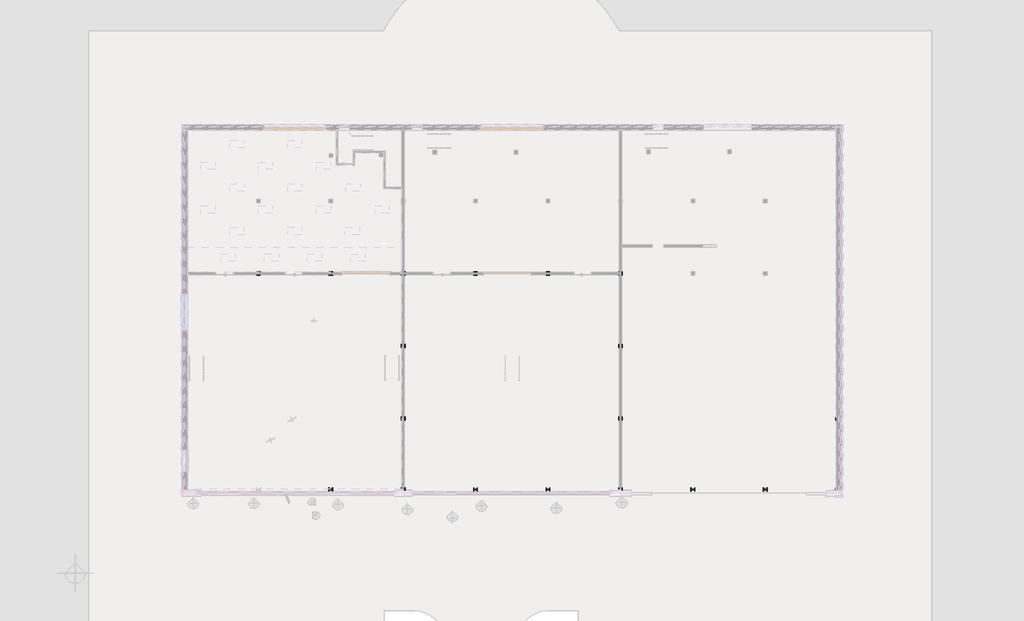
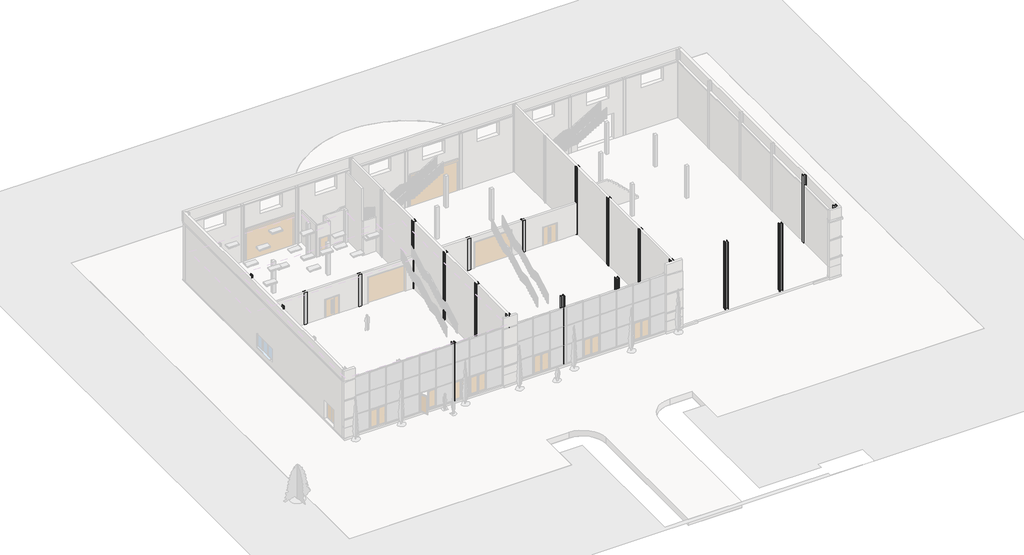
# One storey, part 5 of 13: 21 columns, 21 slabs, 8 footings.
"""IFC4 building model written with IfcOpenShell, lengths in millimetres."""

import ifcopenshell
import ifcopenshell.guid

model = None  # the IFC model being written
_history = None  # IfcOwnerHistory: only IFC2X3 demands one
_inside = {}  # id of a spatial element -> (the spatial element, [elements in it])
_under = {}  # id of a project, library or spatial element -> (it, [spatial elements below it])
_declared = {}  # id of a project -> (the project, [libraries it declares])
_typed = {}  # id of a type object -> (the type object, [elements of that type])
_made_of = {}  # id of a material, layer set ... -> (it, [elements and type objects made of it])


def new_model(schema):
    """Start an empty IFC model of exactly this schema.

    Asked for "IFC4X3", IfcOpenShell would pick the latest addendum, in which some entities
    have other attributes; the version numbers below select the first issue.
    IFC2X3 requires an IfcOwnerHistory on every rooted entity: one is made here for all.
    """
    global model, _history
    if schema == "IFC4X3":
        model = ifcopenshell.file(schema_version=(4, 3, 0, 0))
    else:
        model = ifcopenshell.file(schema=schema)
    _inside.clear()
    _under.clear()
    _declared.clear()
    _typed.clear()
    _made_of.clear()
    _history = None
    if model.schema == "IFC2X3":
        org = make("IfcOrganization", Name="unknown")
        user = make(
            "IfcPersonAndOrganization",
            ThePerson=make("IfcPerson", FamilyName="unknown"),
            TheOrganization=org,
        )
        app = make(
            "IfcApplication",
            ApplicationDeveloper=org,
            Version="unknown",
            ApplicationFullName="unknown",
            ApplicationIdentifier="unknown",
        )
        _history = make(
            "IfcOwnerHistory",
            OwningUser=user,
            OwningApplication=app,
            ChangeAction="ADDED",
            CreationDate=0,
        )
    return model


def make(cls, **values):
    """One entity of the class cls with the attributes given. An attribute that is None is left unset."""
    return model.create_entity(
        cls, **{name: value for name, value in values.items() if value is not None}
    )


def rooted(cls, **values):
    """An entity with a GlobalId (a new one), such as an element, a storey or a relation."""
    return make(cls, GlobalId=ifcopenshell.guid.new(), OwnerHistory=_history, **values)


def si_unit(unit_type, name, prefix=None):
    """IfcSIUnit, for example si_unit("LENGTHUNIT", "METRE", prefix="MILLI")."""
    return make("IfcSIUnit", UnitType=unit_type, Prefix=prefix, Name=name)


def assignment(units):
    """IfcUnitAssignment: the units of a project."""
    return None if units is None else make("IfcUnitAssignment", Units=units)


def point(xyz):
    """IfcCartesianPoint."""
    return None if xyz is None else make("IfcCartesianPoint", Coordinates=xyz)


def direction(xyz):
    """IfcDirection."""
    return None if xyz is None else make("IfcDirection", DirectionRatios=xyz)


def frame(location, z_axis=None, x_axis=None):
    """IfcAxis2Placement3D, a coordinate frame: its origin and axes. An axis left out is left unset."""
    return make(
        "IfcAxis2Placement3D",
        Location=point(location),
        Axis=direction(z_axis),
        RefDirection=direction(x_axis),
    )


def frame_2d(location, x_axis=None):
    """IfcAxis2Placement2D, a coordinate frame in the plane: its origin and x axis."""
    return make(
        "IfcAxis2Placement2D", Location=point(location), RefDirection=direction(x_axis)
    )


def origin():
    """The frame at (0, 0, 0) with its axes left unset."""
    return frame((0.0, 0.0, 0.0))


def place(relative_to, where):
    """IfcLocalPlacement: puts the frame where relative to a parent placement (None: the world)."""
    return make(
        "IfcLocalPlacement", PlacementRelTo=relative_to, RelativePlacement=where
    )


def context(
    kind, dimensions, precision=None, world=None, true_north=None, identifier=None
):
    """IfcGeometricRepresentationContext, for example the 3D "Model" context."""
    return make(
        "IfcGeometricRepresentationContext",
        ContextIdentifier=identifier,
        ContextType=kind,
        CoordinateSpaceDimension=dimensions,
        Precision=precision,
        WorldCoordinateSystem=world,
        TrueNorth=true_north,
    )


def project(units=None, contexts=None):
    """IfcProject with its units and contexts."""
    return rooted(
        "IfcProject",
        Name="project",
        RepresentationContexts=contexts,
        UnitsInContext=assignment(units),
    )


def spatial(cls, under=None, at=None, **own):
    """A site, building, storey or space (cls), placed at a placement, below another one or the project."""
    s = rooted(cls, ObjectPlacement=at, **own)
    if under is not None:
        _under.setdefault(under.id(), (under, []))[1].append(s)
    return s


def polyline(points):
    """IfcPolyline through the points."""
    return make("IfcPolyline", Points=[point(p) for p in points])


def circle_curve(where, radius):
    """IfcCircle in the frame where."""
    return make("IfcCircle", Position=where, Radius=radius)


def trimmed(basis, trim1, trim2, sense, master):
    """IfcTrimmedCurve: the piece of a basis curve between two trims."""
    return make(
        "IfcTrimmedCurve",
        BasisCurve=basis,
        Trim1=trim1,
        Trim2=trim2,
        SenseAgreement=sense,
        MasterRepresentation=master,
    )


def segment(curve, same_sense, transition):
    """IfcCompositeCurveSegment."""
    return make(
        "IfcCompositeCurveSegment",
        Transition=transition,
        SameSense=same_sense,
        ParentCurve=curve,
    )


def composite_curve(segments, self_intersect=None):
    """IfcCompositeCurve: segments joined end to end."""
    return make("IfcCompositeCurve", Segments=segments, SelfIntersect=self_intersect)


def outline(outer, holes=None, kind="AREA"):
    """IfcArbitraryClosedProfileDef: a profile drawn as a closed curve; with holes, ...WithVoids."""
    if holes is None:
        return make("IfcArbitraryClosedProfileDef", ProfileType=kind, OuterCurve=outer)
    return make(
        "IfcArbitraryProfileDefWithVoids",
        ProfileType=kind,
        OuterCurve=outer,
        InnerCurves=holes,
    )


def extrude(swept, where, along, depth):
    """IfcExtrudedAreaSolid: the profile swept, set in the frame where, extruded along a direction by depth."""
    return make(
        "IfcExtrudedAreaSolid",
        SweptArea=swept,
        Position=where,
        ExtrudedDirection=direction(along),
        Depth=depth,
    )


def faces_of(points, faces, orient=None, outer=None):
    """IfcFace entities. A face is a list of loops; a loop is a list of indices into points, from 0.

    orient and outer hold one flag for each loop. By default every Orientation is true, the
    first loop of a face is its IfcFaceOuterBound and the others are IfcFaceBound.
    """
    made = []
    for i, loops in enumerate(faces):
        bounds = []
        for j, loop in enumerate(loops):
            is_outer = j == 0 if outer is None else outer[i][j]
            bounds.append(
                make(
                    "IfcFaceOuterBound" if is_outer else "IfcFaceBound",
                    Bound=make("IfcPolyLoop", Polygon=[points[k] for k in loop]),
                    Orientation=True if orient is None else orient[i][j],
                )
            )
        made.append(make("IfcFace", Bounds=bounds))
    return made


def faceted_brep(points, faces, orient=None, outer=None, voids=None):
    """IfcFacetedBrep: a solid bounded by flat faces; with voids (closed shells), ...WithVoids."""
    shared = [point(p) for p in points]
    hull = make("IfcClosedShell", CfsFaces=faces_of(shared, faces, orient, outer))
    if voids is None:
        return make("IfcFacetedBrep", Outer=hull)
    return make(
        "IfcFacetedBrepWithVoids",
        Outer=hull,
        Voids=[
            make(cls, CfsFaces=faces_of(shared, fs, o, b)) for cls, fs, o, b in voids
        ],
    )


def shape(context_of_items, identifier, shape_type, items):
    """IfcShapeRepresentation: the items that make up one representation, for example the "Body"."""
    return make(
        "IfcShapeRepresentation",
        ContextOfItems=context_of_items,
        RepresentationIdentifier=identifier,
        RepresentationType=shape_type,
        Items=items,
    )


def source(mapping_origin, context_of_items, identifier, shape_type, items):
    """IfcRepresentationMap: a shape defined once, which mapped items show again and again."""
    return make(
        "IfcRepresentationMap",
        MappingOrigin=mapping_origin,
        MappedRepresentation=shape(context_of_items, identifier, shape_type, items),
    )


def transform(
    local_origin,
    x_axis=None,
    y_axis=None,
    z_axis=None,
    scale=None,
    scale2=None,
    scale3=None,
    uniform=True,
):
    """IfcCartesianTransformationOperator3D, or its non-uniform kind. x_axis, y_axis, z_axis: its Axis1, 2, 3."""
    if uniform:
        return make(
            "IfcCartesianTransformationOperator3D",
            Axis1=direction(x_axis),
            Axis2=direction(y_axis),
            LocalOrigin=point(local_origin),
            Scale=scale,
            Axis3=direction(z_axis),
        )
    return make(
        "IfcCartesianTransformationOperator3DnonUniform",
        Axis1=direction(x_axis),
        Axis2=direction(y_axis),
        LocalOrigin=point(local_origin),
        Scale=scale,
        Axis3=direction(z_axis),
        Scale2=scale2,
        Scale3=scale3,
    )


def mapped(mapping_source, mapping_target):
    """IfcMappedItem: shows the shape of a source again, moved by a transform."""
    return make(
        "IfcMappedItem", MappingSource=mapping_source, MappingTarget=mapping_target
    )


def made_of(thing, what):
    """Note that an element or type object is made of a material, layer set ...; save() writes the relation."""
    if what is not None:
        _made_of.setdefault(what.id(), (what, []))[1].append(thing)
    return thing


def element(
    cls,
    number,
    at=None,
    inside=None,
    cuts=None,
    type_object=None,
    material=None,
    context=None,
    identifier="Body",
    shape_type=None,
    held_by="IfcProductDefinitionShape",
    body=None,
    shapes=None,
    **own,
):
    """One element of the class cls, such as IfcWall. Its Tag is "e" and its number.

    at: its placement. inside: the storey or other place that contains it. cuts: it is an
    opening in that element (IfcRelVoidsElement). A single representation is given by context,
    identifier, shape_type and body (its items); several are given by shapes. held_by: the class
    of the entity that holds the representations. save() writes the other relations.
    """
    e = rooted(cls, Tag="e%d" % number, ObjectPlacement=at, **own)
    if body is not None:
        shapes = [shape(context, identifier, shape_type, body)]
    if shapes is not None:
        e.Representation = make(held_by, Representations=shapes)
    if inside is not None:
        _inside.setdefault(inside.id(), (inside, []))[1].append(e)
    if cuts is not None:
        rooted(
            "IfcRelVoidsElement", RelatingBuildingElement=cuts, RelatedOpeningElement=e
        )
    if type_object is not None:
        _typed.setdefault(type_object.id(), (type_object, []))[1].append(e)
    return made_of(e, material)


def aggregate(whole, parts):
    """IfcRelAggregates: a whole, such as a stair, and the parts it consists of."""
    return rooted("IfcRelAggregates", RelatingObject=whole, RelatedObjects=parts)


def save(model, path):
    """Write the relations noted so far, then the file.

    IfcRelAggregates (storeys below a building ...), IfcRelContainedInSpatialStructure (elements
    in a storey), IfcRelDefinesByType, IfcRelAssociatesMaterial and IfcRelDeclares: one each for
    every whole, place, type object, material and project.
    """
    for whole, parts in _under.values():
        aggregate(whole, parts)
    for where, things in _inside.values():
        rooted(
            "IfcRelContainedInSpatialStructure",
            RelatedElements=things,
            RelatingStructure=where,
        )
    for kind, things in _typed.values():
        rooted("IfcRelDefinesByType", RelatedObjects=things, RelatingType=kind)
    for what, things in _made_of.values():
        rooted("IfcRelAssociatesMaterial", RelatedObjects=things, RelatingMaterial=what)
    for by, libraries in _declared.values():
        rooted("IfcRelDeclares", RelatingContext=by, RelatedDefinitions=libraries)
    model.write(path)


def uc_universal_column_column_305x305x97uc_f4bfb62a(model_context):
    return source(origin(), model_context, "Body", "SweptSolid", [
        extrude(outline(composite_curve([segment(polyline([(152.65, 153.95), (152.65, 138.55), (20.15, 138.55)]), True, "CONTINUOUS"), segment(trimmed(circle_curve(frame_2d((20.15, 123.35)), 15.2), [point((20.15, 138.55))], [point((4.95, 123.35))], True, "CARTESIAN"), True, "CONTINUOUS"), segment(polyline([(4.95, 123.35), (4.95, -123.35)]), True, "CONTINUOUS"), segment(trimmed(circle_curve(frame_2d((20.15, -123.35)), 15.2), [point((4.95, -123.35))], [point((20.15, -138.55))], True, "CARTESIAN"), True, "CONTINUOUS"), segment(polyline([(20.15, -138.55), (152.65, -138.55), (152.65, -153.95), (-152.65, -153.95), (-152.65, -138.55), (-20.15, -138.55)]), True, "CONTINUOUS"), segment(trimmed(circle_curve(frame_2d((-20.15, -123.35)), 15.2), [point((-20.15, -138.55))], [point((-4.95, -123.35))], True, "CARTESIAN"), True, "CONTINUOUS"), segment(polyline([(-4.95, -123.35), (-4.95, 123.35)]), True, "CONTINUOUS"), segment(trimmed(circle_curve(frame_2d((-20.15, 123.35)), 15.2), [point((-4.95, 123.35))], [point((-20.15, 138.55))], True, "CARTESIAN"), True, "CONTINUOUS"), segment(polyline([(-20.15, 138.55), (-152.65, 138.55), (-152.65, 153.95), (152.65, 153.95)]), True, "CONTINUOUS")], self_intersect=False)), frame((0.0, 0.0, -1500.0), z_axis=(0.0, 0.0, 1.0), x_axis=(1.0, 0.0, 0.0)), (0.0, 0.0, 1.0), 9300.0),
    ])


def uc_universal_column_column_305x305x97uc_8da79b43(model_context):
    return source(origin(), model_context, "Body", "SweptSolid", [
        extrude(outline(composite_curve([segment(polyline([(152.65, -153.95), (-152.65, -153.95), (-152.65, -138.55), (-20.15, -138.55)]), True, "CONTINUOUS"), segment(trimmed(circle_curve(frame_2d((-20.15, -123.35)), 15.2), [point((-20.15, -138.55))], [point((-4.95, -123.35))], True, "CARTESIAN"), True, "CONTINUOUS"), segment(polyline([(-4.95, -123.35), (-4.95, 123.35)]), True, "CONTINUOUS"), segment(trimmed(circle_curve(frame_2d((-20.15, 123.35)), 15.2), [point((-4.95, 123.35))], [point((-20.15, 138.55))], True, "CARTESIAN"), True, "CONTINUOUS"), segment(polyline([(-20.15, 138.55), (-152.65, 138.55), (-152.65, 153.95), (152.65, 153.95), (152.65, 138.55), (20.15, 138.55)]), True, "CONTINUOUS"), segment(trimmed(circle_curve(frame_2d((20.15, 123.35)), 15.2), [point((20.15, 138.55))], [point((4.95, 123.35))], True, "CARTESIAN"), True, "CONTINUOUS"), segment(polyline([(4.95, 123.35), (4.95, -123.35)]), True, "CONTINUOUS"), segment(trimmed(circle_curve(frame_2d((20.15, -123.35)), 15.2), [point((4.95, -123.35))], [point((20.15, -138.55))], True, "CARTESIAN"), True, "CONTINUOUS"), segment(polyline([(20.15, -138.55), (152.65, -138.55), (152.65, -153.95)]), True, "CONTINUOUS")], self_intersect=False)), frame((0.0, 0.0, -1500.0), z_axis=(0.0, 0.0, 1.0), x_axis=(1.0, 0.0, 0.0)), (0.0, 0.0, 1.0), 9300.0),
    ])


def uc_universal_column_column_305x305x97uc_43a052ce(model_context):
    return source(origin(), model_context, "Body", "SweptSolid", [
        extrude(outline(composite_curve([segment(polyline([(152.65, 153.95), (152.65, 138.55), (20.15, 138.55)]), True, "CONTINUOUS"), segment(trimmed(circle_curve(frame_2d((20.15, 123.35)), 15.2), [point((20.15, 138.55))], [point((4.95, 123.35))], True, "CARTESIAN"), True, "CONTINUOUS"), segment(polyline([(4.95, 123.35), (4.95, -123.35)]), True, "CONTINUOUS"), segment(trimmed(circle_curve(frame_2d((20.15, -123.35)), 15.2), [point((4.95, -123.35))], [point((20.15, -138.55))], True, "CARTESIAN"), True, "CONTINUOUS"), segment(polyline([(20.15, -138.55), (152.65, -138.55), (152.65, -153.95), (-152.65, -153.95), (-152.65, -138.55), (-20.15, -138.55)]), True, "CONTINUOUS"), segment(trimmed(circle_curve(frame_2d((-20.15, -123.35)), 15.2), [point((-20.15, -138.55))], [point((-4.95, -123.35))], True, "CARTESIAN"), True, "CONTINUOUS"), segment(polyline([(-4.95, -123.35), (-4.95, 123.35)]), True, "CONTINUOUS"), segment(trimmed(circle_curve(frame_2d((-20.15, 123.35)), 15.2), [point((-4.95, 123.35))], [point((-20.15, 138.55))], True, "CARTESIAN"), True, "CONTINUOUS"), segment(polyline([(-20.15, 138.55), (-152.65, 138.55), (-152.65, 153.95), (152.65, 153.95)]), True, "CONTINUOUS")], self_intersect=False)), frame((0.0, 0.0, -1500.0), z_axis=(0.0, 0.0, 1.0), x_axis=(1.0, 0.0, 0.0)), (0.0, 0.0, 1.0), 8100.0),
    ])


def pad_foundation_rectangular_1000x1000x500_ed6229e9(model_context):
    return source(origin(), model_context, "Body", "SweptSolid", [
        extrude(outline(polyline([(500.0, 500.0), (500.0, -500.0), (-500.0, -500.0), (-500.0, 500.0), (500.0, 500.0)])), frame((0.0, 0.0, -500.0), z_axis=(0.0, 0.0, 1.0), x_axis=(1.0, 0.0, 0.0)), (0.0, 0.0, 1.0), 500.0),
    ])


model = new_model("IFC4")

# Units and contexts
model_context = context("Model", 3, world=origin())
ifc_project = project(units=[si_unit("LENGTHUNIT", "METRE", prefix="MILLI")], contexts=[model_context])

# Site, building, storey
site = spatial("IfcSite", under=ifc_project)
building = spatial("IfcBuilding", under=site)
storey = spatial("IfcBuildingStorey", under=building, Name="L0 - Ground Floor (Shadows On)", Elevation=0.0)

# Columns
placement = place(None, origin())
element("IfcColumn", 1, ObjectType="Concrete Square : 300 x 300mm", at=placement, inside=storey, context=model_context, shape_type="SweptSolid", body=[
    extrude(outline(polyline([(-989.5553457, -5208.7619082), (-1289.5553457, -5208.7619082), (-1289.5553457, -4908.7619082), (-989.5553457, -4908.7619082), (-989.5553457, -5208.7619082)])), frame((0.0, 0.0, -1500.0), z_axis=(0.0, 0.0, 1.0), x_axis=(1.0, 0.0, 0.0)), (0.0, 0.0, 1.0), 5200.0),
])
element("IfcColumn", 2, ObjectType="Concrete Square : 300 x 300mm", at=placement, inside=storey, context=model_context, shape_type="SweptSolid", body=[
    extrude(outline(polyline([(5010.4446543, -5208.7619082), (4710.4446543, -5208.7619082), (4710.4446543, -4908.7619082), (5010.4446543, -4908.7619082), (5010.4446543, -5208.7619082)])), frame((0.0, 0.0, -1500.0), z_axis=(0.0, 0.0, 1.0), x_axis=(1.0, 0.0, 0.0)), (0.0, 0.0, 1.0), 5200.0),
])
element("IfcColumn", 3, ObjectType="Concrete Square : 300 x 300mm", at=placement, inside=storey, context=model_context, shape_type="SweptSolid", body=[
    extrude(outline(polyline([(17010.4446543, -5208.7619082), (16710.4446543, -5208.7619082), (16710.4446543, -4908.7619082), (17010.4446543, -4908.7619082), (17010.4446543, -5208.7619082)])), frame((0.0, 0.0, -1500.0), z_axis=(0.0, 0.0, 1.0), x_axis=(1.0, 0.0, 0.0)), (0.0, 0.0, 1.0), 5200.0),
])
element("IfcColumn", 4, ObjectType="Concrete Square : 300 x 300mm", at=placement, inside=storey, context=model_context, shape_type="SweptSolid", body=[
    extrude(outline(polyline([(23010.4446543, -5208.7619082), (22710.4446543, -5208.7619082), (22710.4446543, -4908.7619082), (23010.4446543, -4908.7619082), (23010.4446543, -5208.7619082)])), frame((0.0, 0.0, -1500.0), z_axis=(0.0, 0.0, 1.0), x_axis=(1.0, 0.0, 0.0)), (0.0, 0.0, 1.0), 5200.0),
])
element("IfcColumn", 5, ObjectType="UC-Universal Column-Column : 305x305x97UC", at=placement, inside=storey, context=model_context, shape_type="SweptSolid", body=[
    extrude(outline(composite_curve([segment(polyline([(-7293.5053457, -10906.1119082), (-7278.1053457, -10906.1119082), (-7278.1053457, -11038.6119082)]), True, "CONTINUOUS"), segment(trimmed(circle_curve(frame_2d((-7262.9053457, -11038.6119082)), 15.2), [point((-7278.1053457, -11038.6119082))], [point((-7262.9053457, -11053.8119082))], True, "CARTESIAN"), True, "CONTINUOUS"), segment(polyline([(-7262.9053457, -11053.8119082), (-7016.2053457, -11053.8119082)]), True, "CONTINUOUS"), segment(trimmed(circle_curve(frame_2d((-7016.2053457, -11038.6119082)), 15.2), [point((-7016.2053457, -11053.8119082))], [point((-7001.0053457, -11038.6119082))], True, "CARTESIAN"), True, "CONTINUOUS"), segment(polyline([(-7001.0053457, -11038.6119082), (-7001.0053457, -10906.1119082), (-6985.6053457, -10906.1119082), (-6985.6053457, -11211.4119082), (-7001.0053457, -11211.4119082), (-7001.0053457, -11078.9119082)]), True, "CONTINUOUS"), segment(trimmed(circle_curve(frame_2d((-7016.2053457, -11078.9119082)), 15.2), [point((-7001.0053457, -11078.9119082))], [point((-7016.2053457, -11063.7119082))], True, "CARTESIAN"), True, "CONTINUOUS"), segment(polyline([(-7016.2053457, -11063.7119082), (-7262.9053457, -11063.7119082)]), True, "CONTINUOUS"), segment(trimmed(circle_curve(frame_2d((-7262.9053457, -11078.9119082)), 15.2), [point((-7262.9053457, -11063.7119082))], [point((-7278.1053457, -11078.9119082))], True, "CARTESIAN"), True, "CONTINUOUS"), segment(polyline([(-7278.1053457, -11078.9119082), (-7278.1053457, -11211.4119082), (-7293.5053457, -11211.4119082), (-7293.5053457, -10906.1119082)]), True, "CONTINUOUS")], self_intersect=False)), frame((0.0, 0.0, -1500.0), z_axis=(0.0, 0.0, 1.0), x_axis=(1.0, 0.0, 0.0)), (0.0, 0.0, 1.0), 9300.0),
])
element("IfcColumn", 6, ObjectType="UC-Universal Column-Column : 305x305x97UC", at=placement, inside=storey, context=model_context, shape_type="SweptSolid", body=[
    extrude(outline(composite_curve([segment(polyline([(-7293.5053457, -4906.1119082), (-7278.1053457, -4906.1119082), (-7278.1053457, -5038.6119082)]), True, "CONTINUOUS"), segment(trimmed(circle_curve(frame_2d((-7262.9053457, -5038.6119082)), 15.2), [point((-7278.1053457, -5038.6119082))], [point((-7262.9053457, -5053.8119082))], True, "CARTESIAN"), True, "CONTINUOUS"), segment(polyline([(-7262.9053457, -5053.8119082), (-7016.2053457, -5053.8119082)]), True, "CONTINUOUS"), segment(trimmed(circle_curve(frame_2d((-7016.2053457, -5038.6119082)), 15.2), [point((-7016.2053457, -5053.8119082))], [point((-7001.0053457, -5038.6119082))], True, "CARTESIAN"), True, "CONTINUOUS"), segment(polyline([(-7001.0053457, -5038.6119082), (-7001.0053457, -4906.1119082), (-6985.6053457, -4906.1119082), (-6985.6053457, -5211.4119082), (-7001.0053457, -5211.4119082), (-7001.0053457, -5078.9119082)]), True, "CONTINUOUS"), segment(trimmed(circle_curve(frame_2d((-7016.2053457, -5078.9119082)), 15.2), [point((-7001.0053457, -5078.9119082))], [point((-7016.2053457, -5063.7119082))], True, "CARTESIAN"), True, "CONTINUOUS"), segment(polyline([(-7016.2053457, -5063.7119082), (-7262.9053457, -5063.7119082)]), True, "CONTINUOUS"), segment(trimmed(circle_curve(frame_2d((-7262.9053457, -5078.9119082)), 15.2), [point((-7262.9053457, -5063.7119082))], [point((-7278.1053457, -5078.9119082))], True, "CARTESIAN"), True, "CONTINUOUS"), segment(polyline([(-7278.1053457, -5078.9119082), (-7278.1053457, -5211.4119082), (-7293.5053457, -5211.4119082), (-7293.5053457, -4906.1119082)]), True, "CONTINUOUS")], self_intersect=False)), frame((0.0, 0.0, -1500.0), z_axis=(0.0, 0.0, 1.0), x_axis=(1.0, 0.0, 0.0)), (0.0, 0.0, 1.0), 9300.0),
])
uc_universal_column_column_305x305x97uc_shape = uc_universal_column_column_305x305x97uc_f4bfb62a(model_context)
element("IfcColumn", 7, ObjectType="UC-Universal Column-Column : 305x305x97UC", at=placement, inside=storey, context=model_context, shape_type="MappedRepresentation", body=[
    mapped(uc_universal_column_column_305x305x97uc_shape, transform((10860.4446543, -17058.7619082, 0.0), x_axis=(0.0, 1.0, 0.0), y_axis=(-1.0, 0.0, 0.0), z_axis=(0.0, 0.0, 1.0))),
])
element("IfcColumn", 8, ObjectType="UC-Universal Column-Column : 305x305x97UC", at=placement, inside=storey, context=model_context, shape_type="MappedRepresentation", body=[
    mapped(uc_universal_column_column_305x305x97uc_shape, transform((28860.4446543, -17058.7619082, 0.0), x_axis=(0.0, 1.0, 0.0), y_axis=(-1.0, 0.0, 0.0), z_axis=(0.0, 0.0, 1.0))),
])
element("IfcColumn", 9, ObjectType="UC-Universal Column-Column : 305x305x97UC", at=placement, inside=storey, context=model_context, shape_type="MappedRepresentation", body=[
    mapped(uc_universal_column_column_305x305x97uc_shape, transform((10860.4446543, -11058.7619082, 0.0), x_axis=(0.0, 1.0, 0.0), y_axis=(-1.0, 0.0, 0.0), z_axis=(0.0, 0.0, 1.0))),
])
element("IfcColumn", 10, ObjectType="UC-Universal Column-Column : 305x305x97UC", at=placement, inside=storey, context=model_context, shape_type="MappedRepresentation", body=[
    mapped(uc_universal_column_column_305x305x97uc_shape, transform((28860.4446543, -11058.7619082, 0.0), x_axis=(0.0, 1.0, 0.0), y_axis=(-1.0, 0.0, 0.0), z_axis=(0.0, 0.0, 1.0))),
])
element("IfcColumn", 11, ObjectType="UC-Universal Column-Column : 305x305x97UC", at=placement, inside=storey, context=model_context, shape_type="MappedRepresentation", body=[
    mapped(uc_universal_column_column_305x305x97uc_shape, transform((10860.4446543, -5058.7619082, 0.0), x_axis=(0.0, 1.0, 0.0), y_axis=(-1.0, 0.0, 0.0), z_axis=(0.0, 0.0, 1.0))),
])
element("IfcColumn", 12, ObjectType="UC-Universal Column-Column : 305x305x97UC", at=placement, inside=storey, context=model_context, shape_type="MappedRepresentation", body=[
    mapped(uc_universal_column_column_305x305x97uc_shape, transform((28860.4446543, -5058.7619082, 0.0), x_axis=(0.0, 1.0, 0.0), y_axis=(-1.0, 0.0, 0.0), z_axis=(0.0, 0.0, 1.0))),
])
element("IfcColumn", 13, ObjectType="UC-Universal Column-Column : 305x305x97UC", at=placement, inside=storey, context=model_context, shape_type="MappedRepresentation", body=[
    mapped(uc_universal_column_column_305x305x97uc_shape, transform((10860.4446543, -22948.7619082, 0.0), x_axis=(0.0, 1.0, 0.0), y_axis=(-1.0, 0.0, 0.0), z_axis=(0.0, 0.0, 1.0))),
])
element("IfcColumn", 14, ObjectType="UC-Universal Column-Column : 305x305x97UC", at=placement, inside=storey, context=model_context, shape_type="MappedRepresentation", body=[
    mapped(uc_universal_column_column_305x305x97uc_shape, transform((16860.4446543, -22948.7619082, 0.0), x_axis=(0.0, 1.0, 0.0), y_axis=(-1.0, 0.0, 0.0), z_axis=(0.0, 0.0, 1.0))),
])
element("IfcColumn", 15, ObjectType="UC-Universal Column-Column : 305x305x97UC", at=placement, inside=storey, context=model_context, shape_type="MappedRepresentation", body=[
    mapped(uc_universal_column_column_305x305x97uc_shape, transform((22860.4446543, -22948.7619082, 0.0), x_axis=(0.0, 1.0, 0.0), y_axis=(-1.0, 0.0, 0.0), z_axis=(0.0, 0.0, 1.0))),
])
element("IfcColumn", 16, ObjectType="UC-Universal Column-Column : 305x305x97UC", at=placement, inside=storey, context=model_context, shape_type="MappedRepresentation", body=[
    mapped(uc_universal_column_column_305x305x97uc_shape, transform((34860.4446543, -22948.7619082, 0.0), x_axis=(0.0, 1.0, 0.0), y_axis=(-1.0, 0.0, 0.0), z_axis=(0.0, 0.0, 1.0))),
])
element("IfcColumn", 17, ObjectType="UC-Universal Column-Column : 305x305x97UC", at=placement, inside=storey, context=model_context, shape_type="MappedRepresentation", body=[
    mapped(uc_universal_column_column_305x305x97uc_shape, transform((28860.4446543, -22948.7619082, 0.0), x_axis=(0.0, 1.0, 0.0), y_axis=(-1.0, 0.0, 0.0), z_axis=(0.0, 0.0, 1.0))),
])
element("IfcColumn", 18, ObjectType="UC-Universal Column-Column : 305x305x97UC", at=placement, inside=storey, context=model_context, shape_type="MappedRepresentation", body=[
    mapped(uc_universal_column_column_305x305x97uc_shape, transform((40860.4446543, -22948.7619082, 0.0), x_axis=(0.0, 1.0, 0.0), y_axis=(-1.0, 0.0, 0.0), z_axis=(0.0, 0.0, 1.0))),
])
uc_universal_column_column_305x305x97uc_2_shape = uc_universal_column_column_305x305x97uc_8da79b43(model_context)
element("IfcColumn", 19, ObjectType="UC-Universal Column-Column : 305x305x97UC", at=placement, inside=storey, context=model_context, shape_type="MappedRepresentation", body=[
    mapped(uc_universal_column_column_305x305x97uc_2_shape, transform((46860.4446543, -22948.7619082, 0.0), x_axis=(0.0, 1.0, 0.0), y_axis=(-1.0, 0.0, 0.0), z_axis=(0.0, 0.0, 1.0))),
])
element("IfcColumn", 20, ObjectType="UC-Universal Column-Column : 305x305x97UC", at=placement, inside=storey, context=model_context, shape_type="MappedRepresentation", body=[
    mapped(uc_universal_column_column_305x305x97uc_2_shape, transform((46860.4446543, -17058.7619082, 0.0), x_axis=(0.0, 1.0, 0.0), y_axis=(-1.0, 0.0, 0.0), z_axis=(0.0, 0.0, 1.0))),
])
uc_universal_column_column_305x305x97uc_3_shape = uc_universal_column_column_305x305x97uc_43a052ce(model_context)
element("IfcColumn", 21, ObjectType="UC-Universal Column-Column : 305x305x97UC", at=placement, inside=storey, context=model_context, shape_type="MappedRepresentation", body=[
    mapped(uc_universal_column_column_305x305x97uc_3_shape, transform((4860.4446543, -22948.7619082, 0.0), x_axis=(0.0, 1.0, 0.0), y_axis=(-1.0, 0.0, 0.0), z_axis=(0.0, 0.0, 1.0))),
])

# Footings
element("IfcFooting", 22, ObjectType="Wall Foundation - Commercial 1300 x 450", at=placement, inside=storey, context=model_context, shape_type="Brep", body=[
    faceted_brep([(-7673.2053457, 7505.9380918, -1200.0), (-7673.2053457, -23738.4619082, -1200.0), (-6758.8053457, -23738.4619082, -1200.0), (-6758.8053457, -22824.0619082, -1200.0), (-6758.8053457, 6591.5380918, -1200.0), (-6758.8053457, 7505.9380918, -1200.0), (-7673.2053457, 7505.9380918, -1504.8), (-7673.2053457, -23738.4619082, -1504.8), (-6758.8053457, 7505.9380918, -1504.8), (-6758.8053457, 7441.2380918, -1504.8), (-7639.5553457, 7441.2380918, -1504.8), (-7639.5553457, 6441.2380918, -1504.8), (-6758.8053457, 6441.2380918, -1504.8), (-6758.8053457, 1441.2380918, -1504.8), (-7639.5553457, 1441.2380918, -1504.8), (-7639.5553457, 441.2380918, -1504.8), (-6758.8053457, 441.2380918, -1504.8), (-6758.8053457, -4558.7619082, -1504.8), (-7639.5553457, -4558.7619082, -1504.8), (-7639.5553457, -5558.7619082, -1504.8), (-6758.8053457, -5558.7619082, -1504.8), (-6758.8053457, -10558.7619082, -1504.8), (-7639.5553457, -10558.7619082, -1504.8), (-7639.5553457, -11558.7619082, -1504.8), (-6758.8053457, -11558.7619082, -1504.8), (-6758.8053457, -16558.7619082, -1504.8), (-7639.5553457, -16558.7619082, -1504.8), (-7639.5553457, -17558.7619082, -1504.8), (-6758.8053457, -17558.7619082, -1504.8), (-6758.8053457, -22448.7619082, -1504.8), (-7639.5553457, -22448.7619082, -1504.8), (-7639.5553457, -23448.7619082, -1504.8), (-6758.8053457, -23448.7619082, -1504.8), (-6758.8053457, -23738.4619082, -1504.8), (-6758.8053457, -23448.7619082, -1500.0), (-6758.8053457, -22824.0619082, -1500.0), (-6758.8053457, -22448.7619082, -1500.0), (-6758.8053457, -17558.7619082, -1500.0), (-6758.8053457, -16558.7619082, -1500.0), (-6758.8053457, -11558.7619082, -1500.0), (-6758.8053457, -10558.7619082, -1500.0), (-6758.8053457, -5558.7619082, -1500.0), (-6758.8053457, -4558.7619082, -1500.0), (-6758.8053457, 441.2380918, -1500.0), (-6758.8053457, 1441.2380918, -1500.0), (-6758.8053457, 6441.2380918, -1500.0), (-6758.8053457, 6591.5380918, -1500.0), (-6758.8053457, 7441.2380918, -1500.0), (-7639.5553457, 441.2380918, -1500.0), (-7639.5553457, 1441.2380918, -1500.0), (-7639.5553457, 6441.2380918, -1500.0), (-7639.5553457, 7441.2380918, -1500.0), (-7639.5553457, -5558.7619082, -1500.0), (-7639.5553457, -4558.7619082, -1500.0), (-7639.5553457, -11558.7619082, -1500.0), (-7639.5553457, -10558.7619082, -1500.0), (-7639.5553457, -17558.7619082, -1500.0), (-7639.5553457, -16558.7619082, -1500.0), (-7639.5553457, -23448.7619082, -1500.0), (-7639.5553457, -22448.7619082, -1500.0)], [[[0, 1, 2, 3, 4, 5]], [[1, 0, 6, 7]], [[7, 6, 8, 9, 10, 11, 12, 13, 14, 15, 16, 17, 18, 19, 20, 21, 22, 23, 24, 25, 26, 27, 28, 29, 30, 31, 32, 33]], [[5, 4, 3, 2, 33, 32, 34, 35, 36, 29, 28, 37, 38, 25, 24, 39, 40, 21, 20, 41, 42, 17, 16, 43, 44, 13, 12, 45, 46, 47, 9, 8]], [[2, 1, 7, 33]], [[48, 49, 44, 43]], [[44, 49, 14, 13]], [[49, 48, 15, 14]], [[48, 43, 16, 15]], [[50, 51, 47, 46, 45]], [[51, 50, 11, 10]], [[50, 45, 12, 11]], [[52, 53, 42, 41]], [[42, 53, 18, 17]], [[53, 52, 19, 18]], [[52, 41, 20, 19]], [[54, 55, 40, 39]], [[40, 55, 22, 21]], [[55, 54, 23, 22]], [[54, 39, 24, 23]], [[56, 57, 38, 37]], [[38, 57, 26, 25]], [[57, 56, 27, 26]], [[56, 37, 28, 27]], [[58, 59, 36, 35, 34]], [[36, 59, 30, 29]], [[59, 58, 31, 30]], [[0, 5, 8, 6]], [[47, 51, 10, 9]], [[58, 34, 32, 31]]]),
])
element("IfcFooting", 23, ObjectType="Wall Foundation - Commercial 1300 x 450", at=placement, inside=storey, context=model_context, shape_type="Brep", body=[
    faceted_brep([(11600.0976476, -23733.4474846, -1200.0), (11600.0976476, -23733.4474846, -1504.8), (11600.0976476, -23618.4474846, -1504.8), (11600.0976476, -22819.0474846, -1504.8), (11600.0976476, -22819.0474846, -1200.0), (11600.0976476, -23618.4474846, -1200.0), (10120.0976476, -23733.4474846, -1504.8), (10120.0976476, -23733.4474846, -1200.0), (10120.0976476, -23625.2469755, -1200.0), (10120.0976476, -22819.0474846, -1200.0), (10120.0976476, -22819.0474846, -1504.8), (10120.0976476, -23625.2469755, -1504.8), (11317.6446543, -22819.0474846, -1200.0), (10403.2446543, -22819.0474846, -1200.0), (10360.4446543, -22819.0474846, -1504.8), (10360.4446543, -23448.7619082, -1504.8), (11360.4446543, -23448.7619082, -1504.8), (11360.4446543, -22819.0474846, -1504.8), (11360.4446543, -22819.0474846, -1500.0), (11317.6446543, -22819.0474846, -1500.0), (10403.2446543, -22819.0474846, -1500.0), (10360.4446543, -22819.0474846, -1500.0), (11360.4446543, -23448.7619082, -1500.0), (10360.4446543, -23448.7619082, -1500.0)], [[[0, 1, 2, 3, 4, 5]], [[6, 7, 8, 9, 10, 11]], [[7, 0, 5, 4, 12, 13, 9, 8]], [[1, 0, 7, 6]], [[3, 2, 1, 6, 11, 10, 14, 15, 16, 17]], [[4, 3, 17, 18, 19, 20, 21, 14, 10, 9, 13, 12]], [[22, 23, 21, 20, 19, 18]], [[21, 23, 15, 14]], [[23, 22, 16, 15]], [[22, 18, 17, 16]]]),
])
element("IfcFooting", 24, ObjectType="Wall Foundation - Commercial 1300 x 450", at=placement, inside=storey, context=model_context, shape_type="Brep", body=[
    faceted_brep([(31560.0976476, -23733.4474846, -1200.0), (31560.0976476, -23733.4474846, -1504.8), (31560.0976476, -22819.0474846, -1504.8), (31560.0976476, -22819.0474846, -1200.0), (27960.0976476, -23733.4474846, -1504.8), (27960.0976476, -23733.4474846, -1200.0), (27960.0976476, -23618.4474846, -1200.0), (27960.0976476, -22819.0474846, -1200.0), (27960.0976476, -22819.0474846, -1504.8), (27960.0976476, -23618.4474846, -1504.8), (29317.6446543, -22819.0474846, -1200.0), (28403.2446543, -22819.0474846, -1200.0), (28360.4446543, -22819.0474846, -1504.8), (28360.4446543, -23448.7619082, -1504.8), (29360.4446543, -23448.7619082, -1504.8), (29360.4446543, -22819.0474846, -1504.8), (29360.4446543, -22819.0474846, -1500.0), (29317.6446543, -22819.0474846, -1500.0), (28403.2446543, -22819.0474846, -1500.0), (28360.4446543, -22819.0474846, -1500.0), (29360.4446543, -23448.7619082, -1500.0), (28360.4446543, -23448.7619082, -1500.0)], [[[0, 1, 2, 3]], [[4, 5, 6, 7, 8, 9]], [[5, 0, 3, 10, 11, 7, 6]], [[1, 0, 5, 4]], [[2, 1, 4, 9, 8, 12, 13, 14, 15]], [[3, 2, 15, 16, 17, 18, 19, 12, 8, 7, 11, 10]], [[20, 21, 19, 18, 17, 16]], [[19, 21, 13, 12]], [[21, 20, 14, 13]], [[20, 16, 15, 14]]]),
])
element("IfcFooting", 25, ObjectType="Wall Foundation - Commercial 1300 x 450", at=placement, inside=storey, context=model_context, shape_type="Brep", body=[
    faceted_brep([(43960.0976476, -23733.4474846, -1504.8), (43960.0976476, -23733.4474846, -1200.0), (43960.0976476, -22819.0474846, -1200.0), (43960.0976476, -22819.0474846, -1504.8), (47425.1446543, -23733.4474846, -1200.0), (47425.1446543, -22819.0474846, -1200.0), (46510.7446543, -22819.0474846, -1200.0), (47425.1446543, -23733.4474846, -1504.8), (46360.4446543, -22819.0474846, -1504.8), (46360.4446543, -23448.7619082, -1504.8), (47360.4446543, -23448.7619082, -1504.8), (47360.4446543, -22819.0474846, -1504.8), (47425.1446543, -22819.0474846, -1504.8), (47360.4446543, -22819.0474846, -1500.0), (46510.7446543, -22819.0474846, -1500.0), (46360.4446543, -22819.0474846, -1500.0), (47360.4446543, -23448.7619082, -1500.0), (46360.4446543, -23448.7619082, -1500.0)], [[[0, 1, 2, 3]], [[1, 4, 5, 6, 2]], [[1, 0, 7, 4]], [[0, 3, 8, 9, 10, 11, 12, 7]], [[3, 2, 6, 5, 12, 11, 13, 14, 15, 8]], [[16, 17, 15, 14, 13]], [[15, 17, 9, 8]], [[17, 16, 10, 9]], [[5, 4, 7, 12]], [[16, 13, 11, 10]]]),
])
element("IfcFooting", 26, ObjectType="Wall Foundation - Commercial 1300 x 450", at=placement, inside=storey, context=model_context, shape_type="SweptSolid", body=[
    extrude(outline(polyline([(1441.2380918, -1500.0), (441.2380918, -1500.0), (441.2380918, -1504.8), (-4558.7619082, -1504.8), (-4558.7619082, -1500.0), (-5558.7619082, -1500.0), (-5558.7619082, -1504.8), (-10558.7619082, -1504.8), (-10558.7619082, -1500.0), (-11558.7619082, -1500.0), (-11558.7619082, -1504.8), (-16558.7619082, -1504.8), (-16558.7619082, -1500.0), (-17558.7619082, -1500.0), (-17558.7619082, -1504.8), (-22448.7619082, -1504.8), (-22448.7619082, -1500.0), (-22819.0474846, -1500.0), (-22819.0474846, -1200.0), (6591.5380918, -1200.0), (6591.5380918, -1500.0), (6441.2380918, -1500.0), (6441.2380918, -1504.8), (1441.2380918, -1504.8), (1441.2380918, -1500.0)])), frame((28403.2446543, 0.0, 0.0), z_axis=(1.0, 0.0, 0.0), x_axis=(0.0, 1.0, 0.0)), (0.0, 0.0, 1.0), 914.4),
])
element("IfcFooting", 27, ObjectType="Wall Foundation - Commercial 1300 x 450", at=placement, inside=storey, context=model_context, shape_type="SweptSolid", body=[
    extrude(outline(polyline([(1441.2380918, -1500.0), (441.2380918, -1500.0), (441.2380918, -1504.8), (-4558.7619082, -1504.8), (-4558.7619082, -1500.0), (-5558.7619082, -1500.0), (-5558.7619082, -1504.8), (-10558.7619082, -1504.8), (-10558.7619082, -1500.0), (-11558.7619082, -1500.0), (-11558.7619082, -1504.8), (-16558.7619082, -1504.8), (-16558.7619082, -1500.0), (-17558.7619082, -1500.0), (-17558.7619082, -1504.8), (-22448.7619082, -1504.8), (-22448.7619082, -1500.0), (-22819.0474846, -1500.0), (-22819.0474846, -1200.0), (6591.5380918, -1200.0), (6591.5380918, -1500.0), (6441.2380918, -1500.0), (6441.2380918, -1504.8), (1441.2380918, -1504.8), (1441.2380918, -1500.0)])), frame((10403.2446543, 0.0, 0.0), z_axis=(1.0, 0.0, 0.0), x_axis=(0.0, 1.0, 0.0)), (0.0, 0.0, 1.0), 914.4),
])
element("IfcFooting", 28, ObjectType="Wall Foundation - Commercial 1300 x 450", at=placement, inside=storey, context=model_context, shape_type="Brep", body=[
    faceted_brep([(-6531.0053457, -22710.8469755, -1200.0), (-6531.0053457, -22710.8469755, -1504.8), (-6531.0053457, -22824.0619082, -1504.8), (-6531.0053457, -23625.2469755, -1504.8), (-6531.0053457, -23625.2469755, -1200.0), (-6531.0053457, -22824.0619082, -1200.0), (10120.0976476, -22710.8469755, -1504.8), (10120.0976476, -22710.8469755, -1200.0), (10120.0976476, -22819.0474846, -1200.0), (10120.0976476, -23625.2469755, -1200.0), (10120.0976476, -23625.2469755, -1504.8), (10120.0976476, -22819.0474846, -1504.8), (-6239.5553457, -23625.2469755, -1200.0), (-6214.1553457, -23625.2469755, -1200.0), (-6214.1553457, -22824.0619082, -1200.0), (-5856.0053457, -22824.0619082, -1200.0), (-5856.0053457, -23625.2469755, -1200.0), (5360.4446543, -22710.8469755, -1504.8), (5360.4446543, -22710.8469755, -1500.0), (4360.4446543, -22710.8469755, -1500.0), (4360.4446543, -22710.8469755, -1504.8), (-639.5553457, -22710.8469755, -1504.8), (-639.5553457, -22710.8469755, -1500.0), (-1639.5553457, -22710.8469755, -1500.0), (-1639.5553457, -22710.8469755, -1504.8), (-1639.5553457, -23448.7619082, -1504.8), (-639.5553457, -23448.7619082, -1504.8), (4360.4446543, -23448.7619082, -1504.8), (5360.4446543, -23448.7619082, -1504.8), (-5856.0053457, -23625.2469755, -1504.8), (-5856.0053457, -22824.0619082, -1504.8), (-6214.1553457, -22824.0619082, -1504.8), (-6214.1553457, -23625.2469755, -1504.8), (-6239.5553457, -23625.2469755, -1504.8), (5360.4446543, -23448.7619082, -1500.0), (4360.4446543, -23448.7619082, -1500.0), (-639.5553457, -23448.7619082, -1500.0), (-1639.5553457, -23448.7619082, -1500.0)], [[[0, 1, 2, 3, 4, 5]], [[6, 7, 8, 9, 10, 11]], [[7, 0, 5, 4, 12, 13, 14, 15, 16, 9, 8]], [[1, 0, 7, 6, 17, 18, 19, 20, 21, 22, 23, 24]], [[3, 2, 1, 24, 25, 26, 21, 20, 27, 28, 17, 6, 11, 10, 29, 30, 31, 32, 33]], [[10, 9, 16, 29]], [[4, 3, 33, 32, 13, 12]], [[34, 35, 19, 18]], [[19, 35, 27, 20]], [[35, 34, 28, 27]], [[34, 18, 17, 28]], [[36, 37, 23, 22]], [[23, 37, 25, 24]], [[37, 36, 26, 25]], [[36, 22, 21, 26]], [[15, 30, 29, 16]], [[30, 15, 14, 31]], [[31, 14, 13, 32]]]),
])
element("IfcFooting", 29, ObjectType="Wall Foundation - Commercial 1300 x 450", at=placement, inside=storey, context=model_context, shape_type="Brep", body=[
    faceted_brep([(27960.0976476, -23618.4474846, -1200.0), (27960.0976476, -23618.4474846, -1504.8), (27960.0976476, -22819.0474846, -1504.8), (27960.0976476, -22704.0474846, -1504.8), (27960.0976476, -22704.0474846, -1200.0), (27960.0976476, -22819.0474846, -1200.0), (11600.0976476, -23618.4474846, -1504.8), (11600.0976476, -23618.4474846, -1200.0), (11600.0976476, -22819.0474846, -1200.0), (11600.0976476, -22704.0474846, -1200.0), (11600.0976476, -22704.0474846, -1504.8), (11600.0976476, -22819.0474846, -1504.8), (16360.4446543, -22704.0474846, -1504.8), (16360.4446543, -23448.7619082, -1504.8), (17360.4446543, -23448.7619082, -1504.8), (17360.4446543, -22704.0474846, -1504.8), (22360.4446543, -22704.0474846, -1504.8), (22360.4446543, -23448.7619082, -1504.8), (23360.4446543, -23448.7619082, -1504.8), (23360.4446543, -22704.0474846, -1504.8), (23360.4446543, -22704.0474846, -1500.0), (22360.4446543, -22704.0474846, -1500.0), (17360.4446543, -22704.0474846, -1500.0), (16360.4446543, -22704.0474846, -1500.0), (23360.4446543, -23448.7619082, -1500.0), (22360.4446543, -23448.7619082, -1500.0), (17360.4446543, -23448.7619082, -1500.0), (16360.4446543, -23448.7619082, -1500.0)], [[[0, 1, 2, 3, 4, 5]], [[6, 7, 8, 9, 10, 11]], [[7, 0, 5, 4, 9, 8]], [[1, 0, 7, 6]], [[3, 2, 1, 6, 11, 10, 12, 13, 14, 15, 16, 17, 18, 19]], [[4, 3, 19, 20, 21, 16, 15, 22, 23, 12, 10, 9]], [[24, 25, 21, 20]], [[21, 25, 17, 16]], [[25, 24, 18, 17]], [[24, 20, 19, 18]], [[26, 27, 23, 22]], [[23, 27, 13, 12]], [[27, 26, 14, 13]], [[26, 22, 15, 14]]]),
])

# Slabs
element("IfcSlab", 30, ObjectType="Pad Foundation-Rectangular : 1000x1000x500", at=placement, inside=storey, context=model_context, shape_type="Brep", body=[
    faceted_brep([(11360.4446543, -4558.7619082, -1500.0), (11317.6446543, -4558.7619082, -1500.0), (10403.2446543, -4558.7619082, -1500.0), (10360.4446543, -4558.7619082, -1500.0), (10360.4446543, -5558.7619082, -1500.0), (10403.2446543, -5558.7619082, -1500.0), (11317.6446543, -5558.7619082, -1500.0), (11360.4446543, -5558.7619082, -1500.0), (11360.4446543, -4558.7619082, -2000.0), (11360.4446543, -5558.7619082, -2000.0), (10360.4446543, -5558.7619082, -2000.0), (10360.4446543, -4558.7619082, -2000.0)], [[[0, 1, 2, 3, 4, 5, 6, 7]], [[8, 9, 10, 11]], [[3, 2, 1, 0, 8, 11]], [[4, 3, 11, 10]], [[7, 6, 5, 4, 10, 9]], [[0, 7, 9, 8]]]),
])
element("IfcSlab", 31, ObjectType="Pad Foundation-Rectangular : 1000x1000x500", at=placement, inside=storey, context=model_context, shape_type="Brep", body=[
    faceted_brep([(29360.4446543, -4558.7619082, -1500.0), (29317.6446543, -4558.7619082, -1500.0), (28403.2446543, -4558.7619082, -1500.0), (28360.4446543, -4558.7619082, -1500.0), (28360.4446543, -5558.7619082, -1500.0), (28403.2446543, -5558.7619082, -1500.0), (29317.6446543, -5558.7619082, -1500.0), (29360.4446543, -5558.7619082, -1500.0), (29360.4446543, -4558.7619082, -2000.0), (29360.4446543, -5558.7619082, -2000.0), (28360.4446543, -5558.7619082, -2000.0), (28360.4446543, -4558.7619082, -2000.0)], [[[0, 1, 2, 3, 4, 5, 6, 7]], [[8, 9, 10, 11]], [[3, 2, 1, 0, 8, 11]], [[4, 3, 11, 10]], [[7, 6, 5, 4, 10, 9]], [[0, 7, 9, 8]]]),
])
element("IfcSlab", 32, ObjectType="Pad Foundation-Rectangular : 1000x1000x500", at=placement, inside=storey, context=model_context, shape_type="Brep", body=[
    faceted_brep([(-6639.5553457, -4558.7619082, -1500.0), (-6758.8053457, -4558.7619082, -1500.0), (-7639.5553457, -4558.7619082, -1500.0), (-7639.5553457, -5558.7619082, -1500.0), (-6758.8053457, -5558.7619082, -1500.0), (-6639.5553457, -5558.7619082, -1500.0), (-6639.5553457, -4558.7619082, -2000.0), (-6639.5553457, -5558.7619082, -2000.0), (-7639.5553457, -5558.7619082, -2000.0), (-7639.5553457, -4558.7619082, -2000.0), (-7639.5553457, -4558.7619082, -1504.8), (-7639.5553457, -5558.7619082, -1504.8)], [[[0, 1, 2, 3, 4, 5]], [[6, 7, 8, 9]], [[2, 1, 0, 6, 9, 10]], [[3, 2, 10, 9, 8, 11]], [[5, 4, 3, 11, 8, 7]], [[0, 5, 7, 6]]]),
])
element("IfcSlab", 33, ObjectType="Pad Foundation-Rectangular : 1000x1000x500", at=placement, inside=storey, context=model_context, shape_type="Brep", body=[
    faceted_brep([(11360.4446543, -10558.7619082, -1500.0), (11317.6446543, -10558.7619082, -1500.0), (10403.2446543, -10558.7619082, -1500.0), (10360.4446543, -10558.7619082, -1500.0), (10360.4446543, -11558.7619082, -1500.0), (10403.2446543, -11558.7619082, -1500.0), (11317.6446543, -11558.7619082, -1500.0), (11360.4446543, -11558.7619082, -1500.0), (11360.4446543, -10558.7619082, -2000.0), (11360.4446543, -11558.7619082, -2000.0), (10360.4446543, -11558.7619082, -2000.0), (10360.4446543, -10558.7619082, -2000.0)], [[[0, 1, 2, 3, 4, 5, 6, 7]], [[8, 9, 10, 11]], [[3, 2, 1, 0, 8, 11]], [[4, 3, 11, 10]], [[7, 6, 5, 4, 10, 9]], [[0, 7, 9, 8]]]),
])
element("IfcSlab", 34, ObjectType="Pad Foundation-Rectangular : 1000x1000x500", at=placement, inside=storey, context=model_context, shape_type="Brep", body=[
    faceted_brep([(29360.4446543, -10558.7619082, -1500.0), (29317.6446543, -10558.7619082, -1500.0), (28403.2446543, -10558.7619082, -1500.0), (28360.4446543, -10558.7619082, -1500.0), (28360.4446543, -11558.7619082, -1500.0), (28403.2446543, -11558.7619082, -1500.0), (29317.6446543, -11558.7619082, -1500.0), (29360.4446543, -11558.7619082, -1500.0), (29360.4446543, -10558.7619082, -2000.0), (29360.4446543, -11558.7619082, -2000.0), (28360.4446543, -11558.7619082, -2000.0), (28360.4446543, -10558.7619082, -2000.0)], [[[0, 1, 2, 3, 4, 5, 6, 7]], [[8, 9, 10, 11]], [[3, 2, 1, 0, 8, 11]], [[4, 3, 11, 10]], [[7, 6, 5, 4, 10, 9]], [[0, 7, 9, 8]]]),
])
element("IfcSlab", 35, ObjectType="Pad Foundation-Rectangular : 1000x1000x500", at=placement, inside=storey, context=model_context, shape_type="Brep", body=[
    faceted_brep([(-6639.5553457, -10558.7619082, -1500.0), (-6758.8053457, -10558.7619082, -1500.0), (-7639.5553457, -10558.7619082, -1500.0), (-7639.5553457, -11558.7619082, -1500.0), (-6758.8053457, -11558.7619082, -1500.0), (-6639.5553457, -11558.7619082, -1500.0), (-6639.5553457, -10558.7619082, -2000.0), (-6639.5553457, -11558.7619082, -2000.0), (-7639.5553457, -11558.7619082, -2000.0), (-7639.5553457, -10558.7619082, -2000.0), (-7639.5553457, -10558.7619082, -1504.8), (-7639.5553457, -11558.7619082, -1504.8)], [[[0, 1, 2, 3, 4, 5]], [[6, 7, 8, 9]], [[2, 1, 0, 6, 9, 10]], [[3, 2, 10, 9, 8, 11]], [[5, 4, 3, 11, 8, 7]], [[0, 5, 7, 6]]]),
])
element("IfcSlab", 36, ObjectType="Pad Foundation-Rectangular : 1000x1000x500", at=placement, inside=storey, context=model_context, shape_type="Brep", body=[
    faceted_brep([(11360.4446543, -16558.7619082, -1500.0), (11317.6446543, -16558.7619082, -1500.0), (10403.2446543, -16558.7619082, -1500.0), (10360.4446543, -16558.7619082, -1500.0), (10360.4446543, -17558.7619082, -1500.0), (10403.2446543, -17558.7619082, -1500.0), (11317.6446543, -17558.7619082, -1500.0), (11360.4446543, -17558.7619082, -1500.0), (11360.4446543, -16558.7619082, -2000.0), (11360.4446543, -17558.7619082, -2000.0), (10360.4446543, -17558.7619082, -2000.0), (10360.4446543, -16558.7619082, -2000.0)], [[[0, 1, 2, 3, 4, 5, 6, 7]], [[8, 9, 10, 11]], [[3, 2, 1, 0, 8, 11]], [[4, 3, 11, 10]], [[7, 6, 5, 4, 10, 9]], [[0, 7, 9, 8]]]),
])
element("IfcSlab", 37, ObjectType="Pad Foundation-Rectangular : 1000x1000x500", at=placement, inside=storey, context=model_context, shape_type="Brep", body=[
    faceted_brep([(29360.4446543, -16558.7619082, -1500.0), (29317.6446543, -16558.7619082, -1500.0), (28403.2446543, -16558.7619082, -1500.0), (28360.4446543, -16558.7619082, -1500.0), (28360.4446543, -17558.7619082, -1500.0), (28403.2446543, -17558.7619082, -1500.0), (29317.6446543, -17558.7619082, -1500.0), (29360.4446543, -17558.7619082, -1500.0), (29360.4446543, -16558.7619082, -2000.0), (29360.4446543, -17558.7619082, -2000.0), (28360.4446543, -17558.7619082, -2000.0), (28360.4446543, -16558.7619082, -2000.0)], [[[0, 1, 2, 3, 4, 5, 6, 7]], [[8, 9, 10, 11]], [[3, 2, 1, 0, 8, 11]], [[4, 3, 11, 10]], [[7, 6, 5, 4, 10, 9]], [[0, 7, 9, 8]]]),
])
element("IfcSlab", 38, ObjectType="Pad Foundation-Rectangular : 1000x1000x500", at=placement, inside=storey, context=model_context, shape_type="Brep", body=[
    faceted_brep([(-6639.5553457, -16558.7619082, -1500.0), (-6758.8053457, -16558.7619082, -1500.0), (-7639.5553457, -16558.7619082, -1500.0), (-7639.5553457, -17558.7619082, -1500.0), (-6758.8053457, -17558.7619082, -1500.0), (-6639.5553457, -17558.7619082, -1500.0), (-6639.5553457, -16558.7619082, -2000.0), (-6639.5553457, -17558.7619082, -2000.0), (-7639.5553457, -17558.7619082, -2000.0), (-7639.5553457, -16558.7619082, -2000.0), (-7639.5553457, -16558.7619082, -1504.8), (-7639.5553457, -17558.7619082, -1504.8)], [[[0, 1, 2, 3, 4, 5]], [[6, 7, 8, 9]], [[2, 1, 0, 6, 9, 10]], [[3, 2, 10, 9, 8, 11]], [[5, 4, 3, 11, 8, 7]], [[0, 5, 7, 6]]]),
])
element("IfcSlab", 39, ObjectType="Pad Foundation-Rectangular : 1000x1000x500", at=placement, inside=storey, context=model_context, shape_type="SweptSolid", body=[
    extrude(outline(polyline([(41381.4946543, -22448.7619082), (41381.4946543, -23448.7619082), (40381.4946543, -23448.7619082), (40381.4946543, -22448.7619082), (41381.4946543, -22448.7619082)])), frame((0.0, 0.0, -2000.0), z_axis=(0.0, 0.0, 1.0), x_axis=(1.0, 0.0, 0.0)), (0.0, 0.0, 1.0), 500.0),
])
element("IfcSlab", 40, ObjectType="Pad Foundation-Rectangular : 1000x1000x500", at=placement, inside=storey, context=model_context, shape_type="SweptSolid", body=[
    extrude(outline(polyline([(35367.9446543, -22448.7619082), (35367.9446543, -23448.7619082), (34367.9446543, -23448.7619082), (34367.9446543, -22448.7619082), (35367.9446543, -22448.7619082)])), frame((0.0, 0.0, -2000.0), z_axis=(0.0, 0.0, 1.0), x_axis=(1.0, 0.0, 0.0)), (0.0, 0.0, 1.0), 500.0),
])
element("IfcSlab", 41, ObjectType="Pad Foundation-Rectangular : 1000x1000x500", at=placement, inside=storey, context=model_context, shape_type="Brep", body=[
    faceted_brep([(29360.4446543, -22448.7619082, -1500.0), (29317.6446543, -22448.7619082, -1500.0), (28403.2446543, -22448.7619082, -1500.0), (28360.4446543, -22448.7619082, -1500.0), (28360.4446543, -22819.0474846, -1500.0), (28360.4446543, -23448.7619082, -1500.0), (29360.4446543, -23448.7619082, -1500.0), (29360.4446543, -22819.0474846, -1500.0), (29360.4446543, -22448.7619082, -2000.0), (29360.4446543, -23448.7619082, -2000.0), (28360.4446543, -23448.7619082, -2000.0), (28360.4446543, -22448.7619082, -2000.0), (28360.4446543, -23448.7619082, -1504.8), (29360.4446543, -23448.7619082, -1504.8)], [[[0, 1, 2, 3, 4, 5, 6, 7]], [[8, 9, 10, 11]], [[3, 2, 1, 0, 8, 11]], [[5, 4, 3, 11, 10, 12]], [[6, 5, 12, 10, 9, 13]], [[0, 7, 6, 13, 9, 8]]]),
])
element("IfcSlab", 42, ObjectType="Pad Foundation-Rectangular : 1000x1000x500", at=placement, inside=storey, context=model_context, shape_type="Brep", body=[
    faceted_brep([(23360.4446543, -22448.7619082, -1500.0), (22360.4446543, -22448.7619082, -1500.0), (22360.4446543, -22704.0474846, -1500.0), (22360.4446543, -23448.7619082, -1500.0), (23360.4446543, -23448.7619082, -1500.0), (23360.4446543, -22704.0474846, -1500.0), (23360.4446543, -22448.7619082, -2000.0), (23360.4446543, -23448.7619082, -2000.0), (22360.4446543, -23448.7619082, -2000.0), (22360.4446543, -22448.7619082, -2000.0), (22360.4446543, -23448.7619082, -1504.8), (23360.4446543, -23448.7619082, -1504.8)], [[[0, 1, 2, 3, 4, 5]], [[6, 7, 8, 9]], [[1, 0, 6, 9]], [[3, 2, 1, 9, 8, 10]], [[4, 3, 10, 8, 7, 11]], [[0, 5, 4, 11, 7, 6]]]),
])
element("IfcSlab", 43, ObjectType="Pad Foundation-Rectangular : 1000x1000x500", at=placement, inside=storey, context=model_context, shape_type="Brep", body=[
    faceted_brep([(17360.4446543, -22448.7619082, -1500.0), (16360.4446543, -22448.7619082, -1500.0), (16360.4446543, -22704.0474846, -1500.0), (16360.4446543, -23448.7619082, -1500.0), (17360.4446543, -23448.7619082, -1500.0), (17360.4446543, -22704.0474846, -1500.0), (17360.4446543, -22448.7619082, -2000.0), (17360.4446543, -23448.7619082, -2000.0), (16360.4446543, -23448.7619082, -2000.0), (16360.4446543, -22448.7619082, -2000.0), (16360.4446543, -23448.7619082, -1504.8), (17360.4446543, -23448.7619082, -1504.8)], [[[0, 1, 2, 3, 4, 5]], [[6, 7, 8, 9]], [[1, 0, 6, 9]], [[3, 2, 1, 9, 8, 10]], [[4, 3, 10, 8, 7, 11]], [[0, 5, 4, 11, 7, 6]]]),
])
element("IfcSlab", 44, ObjectType="Pad Foundation-Rectangular : 1000x1000x500", at=placement, inside=storey, context=model_context, shape_type="Brep", body=[
    faceted_brep([(11360.4446543, -22448.7619082, -1500.0), (11317.6446543, -22448.7619082, -1500.0), (10403.2446543, -22448.7619082, -1500.0), (10360.4446543, -22448.7619082, -1500.0), (10360.4446543, -22819.0474846, -1500.0), (10360.4446543, -23448.7619082, -1500.0), (11360.4446543, -23448.7619082, -1500.0), (11360.4446543, -22819.0474846, -1500.0), (11360.4446543, -22448.7619082, -2000.0), (11360.4446543, -23448.7619082, -2000.0), (10360.4446543, -23448.7619082, -2000.0), (10360.4446543, -22448.7619082, -2000.0), (10360.4446543, -23448.7619082, -1504.8), (11360.4446543, -23448.7619082, -1504.8)], [[[0, 1, 2, 3, 4, 5, 6, 7]], [[8, 9, 10, 11]], [[3, 2, 1, 0, 8, 11]], [[5, 4, 3, 11, 10, 12]], [[6, 5, 12, 10, 9, 13]], [[0, 7, 6, 13, 9, 8]]]),
])
element("IfcSlab", 45, ObjectType="Pad Foundation-Rectangular : 1000x1000x500", at=placement, inside=storey, context=model_context, shape_type="Brep", body=[
    faceted_brep([(5360.4446543, -22448.7619082, -1500.0), (4360.4446543, -22448.7619082, -1500.0), (4360.4446543, -22710.8469755, -1500.0), (4360.4446543, -23448.7619082, -1500.0), (5360.4446543, -23448.7619082, -1500.0), (5360.4446543, -22710.8469755, -1500.0), (5360.4446543, -22448.7619082, -2000.0), (5360.4446543, -23448.7619082, -2000.0), (4360.4446543, -23448.7619082, -2000.0), (4360.4446543, -22448.7619082, -2000.0), (4360.4446543, -23448.7619082, -1504.8), (5360.4446543, -23448.7619082, -1504.8)], [[[0, 1, 2, 3, 4, 5]], [[6, 7, 8, 9]], [[1, 0, 6, 9]], [[3, 2, 1, 9, 8, 10]], [[4, 3, 10, 8, 7, 11]], [[0, 5, 4, 11, 7, 6]]]),
])
element("IfcSlab", 46, ObjectType="Pad Foundation-Rectangular : 1000x1000x500", at=placement, inside=storey, context=model_context, shape_type="Brep", body=[
    faceted_brep([(47360.4446543, -22448.7619082, -1500.0), (46510.7446543, -22448.7619082, -1500.0), (46360.4446543, -22448.7619082, -1500.0), (46360.4446543, -22819.0474846, -1500.0), (46360.4446543, -23448.7619082, -1500.0), (47360.4446543, -23448.7619082, -1500.0), (47360.4446543, -22819.0474846, -1500.0), (47360.4446543, -22448.7619082, -2000.0), (47360.4446543, -23448.7619082, -2000.0), (46360.4446543, -23448.7619082, -2000.0), (46360.4446543, -22448.7619082, -2000.0), (47360.4446543, -22448.7619082, -1504.8), (46360.4446543, -23448.7619082, -1504.8), (47360.4446543, -23448.7619082, -1504.8)], [[[0, 1, 2, 3, 4, 5, 6]], [[7, 8, 9, 10]], [[2, 1, 0, 11, 7, 10]], [[4, 3, 2, 10, 9, 12]], [[5, 4, 12, 9, 8, 13]], [[0, 6, 5, 13, 8, 7, 11]]]),
])
pad_foundation_rectangular_1000x1000x500_shape = pad_foundation_rectangular_1000x1000x500_ed6229e9(model_context)
element("IfcSlab", 47, ObjectType="Pad Foundation-Rectangular : 1000x1000x500", at=placement, inside=storey, context=model_context, shape_type="MappedRepresentation", body=[
    mapped(pad_foundation_rectangular_1000x1000x500_shape, transform((-1139.5553457, -5058.7619082, -1500.0), x_axis=(1.0, 0.0, 0.0), y_axis=(0.0, 1.0, 0.0), z_axis=(0.0, 0.0, 1.0))),
])
element("IfcSlab", 48, ObjectType="Pad Foundation-Rectangular : 1000x1000x500", at=placement, inside=storey, context=model_context, shape_type="MappedRepresentation", body=[
    mapped(pad_foundation_rectangular_1000x1000x500_shape, transform((4860.4446543, -5058.7619082, -1500.0), x_axis=(1.0, 0.0, 0.0), y_axis=(0.0, 1.0, 0.0), z_axis=(0.0, 0.0, 1.0))),
])
element("IfcSlab", 49, ObjectType="Pad Foundation-Rectangular : 1000x1000x500", at=placement, inside=storey, context=model_context, shape_type="MappedRepresentation", body=[
    mapped(pad_foundation_rectangular_1000x1000x500_shape, transform((16860.4446543, -5058.7619082, -1500.0), x_axis=(1.0, 0.0, 0.0), y_axis=(0.0, 1.0, 0.0), z_axis=(0.0, 0.0, 1.0))),
])
element("IfcSlab", 50, ObjectType="Pad Foundation-Rectangular : 1000x1000x500", at=placement, inside=storey, context=model_context, shape_type="MappedRepresentation", body=[
    mapped(pad_foundation_rectangular_1000x1000x500_shape, transform((22860.4446543, -5058.7619082, -1500.0), x_axis=(1.0, 0.0, 0.0), y_axis=(0.0, 1.0, 0.0), z_axis=(0.0, 0.0, 1.0))),
])

save(model, "model.ifc")

# Revit data of these elements
# Project information
#   Project Status = "Project Status"
#   Client Name = "Revit Project"
#   Project Address = "LIMERICK INSTITUTE of TECHNOLOGY"
#   Project Name = "Commercial Units"
#   Project Number = "01"
# Grids (mm)
#   "A": line (-7587.705, 6941.238) -> (47341.061, 6941.238)
#   "B": line (-7587.705, 941.238) -> (47341.061, 941.238)
#   "C": line (-7587.705, -5058.762) -> (47341.061, -5058.762)
#   "1": line (-7139.555, -23439.181) -> (-7139.555, 8028.559)
#   "2": line (-1139.555, -23439.181) -> (-1139.555, 8028.559)
#   "3": line (4860.445, -23439.181) -> (4860.445, 8028.559)
#   "4": line (10860.445, -23439.181) -> (10860.445, 8028.559)
#   "5": line (16860.445, -23439.181) -> (16860.445, 8028.559)
#   "6": line (22860.445, -23439.181) -> (22860.445, 8028.559)
#   "7": line (28860.445, -23439.181) -> (28860.445, 8028.559)
#   "8": line (34860.445, -23439.181) -> (34860.445, 8028.559)
